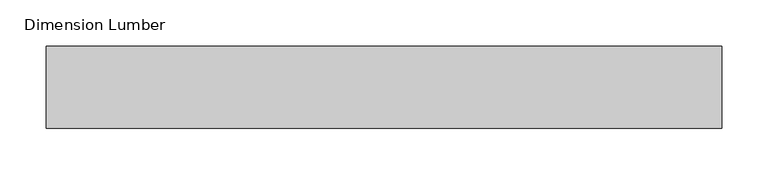
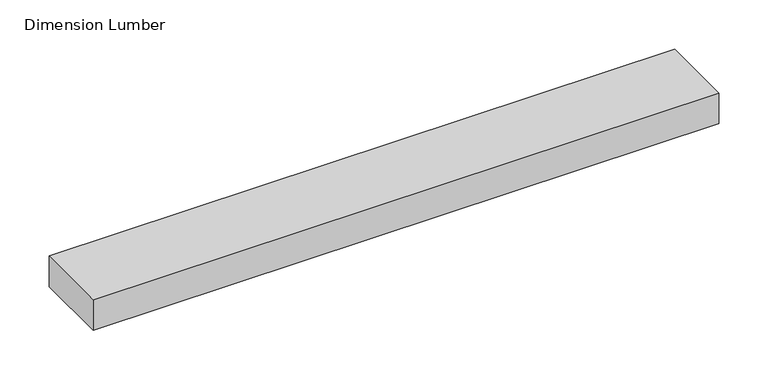
"""IFC4 building model written with IfcOpenShell, lengths in millimetres: beam geometry, Dimension Lumber : Top Supporting Lumbers."""

from ifc_helpers import new_model, si_unit, frame, origin, place, context, project, spatial, polyline, outline, extrude, source, transform, mapped, element, save


def dimension_lumber_d9c95be3(model_context):
    return source(origin(), model_context, "Body", "SweptSolid", [
        extrude(outline(polyline([(346.075, 44.45), (346.075, -44.45), (-384.175, -44.45), (-384.175, 44.45), (346.075, 44.45)])), frame((0.0, 0.0, -19.05), z_axis=(0.0, 0.0, 1.0), x_axis=(1.0, 0.0, 0.0)), (0.0, 0.0, 1.0), 38.1),
    ])


if __name__ == "__main__":
    model = new_model("IFC4")
    model_context = context("Model", 3, world=origin())
    ifc_project = project(units=[si_unit("LENGTHUNIT", "METRE", prefix="MILLI")], contexts=[model_context])
    site = spatial("IfcSite", under=ifc_project)
    building = spatial("IfcBuilding", under=site)
    placement = place(None, origin())
    dimension_lumber_shape = dimension_lumber_d9c95be3(model_context)
    element("IfcBeam", 1, ObjectType="Dimension Lumber : Top Supporting Lumbers", at=placement, inside=building, context=model_context, shape_type="MappedRepresentation", body=[
        mapped(dimension_lumber_shape, transform((0.0, 0.0, 0.0), x_axis=(1.0, 0.0, 0.0), y_axis=(0.0, 1.0, 0.0), z_axis=(0.0, 0.0, 1.0))),
    ])
    save(model, "model.ifc")

# Revit data of these elements
# Type "Dimension Lumber : Top Supporting Lumbers"
#   Assembly Code = "B10"
#   A = 0.0364583 SF
#   Length [instance default] = 5' - 0"
#   b = 0' - 3 1/2"
#   d = 0' - 1 1/2"
#   Structural Material [instance default] = Softwood, Lumber
# Element 1 (IfcBeam, "Dimension Lumber : Top Supporting Lumbers")
#   Structural Material = Douglas Fir #2
#   Materials on its faces: "Douglas Fir #2"
# Materials
#   "Softwood, Lumber": class "Wood", colour RGB 223 192 134, transparency 0, Description = "Pinus Echinata", Cost = 0
#   "Douglas Fir #2": class "Wood", colour RGB 223 192 134, transparency 0, Description = "Pinus Echinata", Cost = 0
